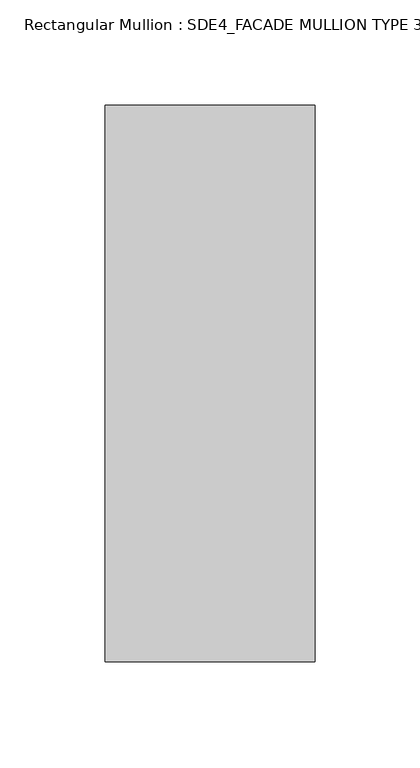
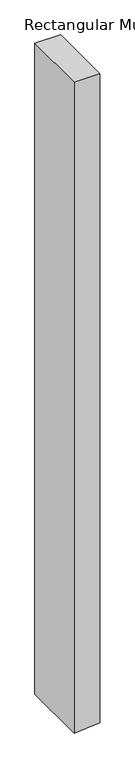
"""IFC4 building model written with IfcOpenShell, lengths in millimetres: member geometry, Rectangular Mullion : SDE4_FACADE MULLION TYPE 3."""

from ifc_helpers import new_model, si_unit, frame, origin, place, context, project, spatial, polyline, outline, extrude, source, transform, mapped, element, save


def rectangular_mullion_sde4_facade_mullion_type_3_780f94bb(model_context):
    return source(origin(), model_context, "Body", "SweptSolid", [
        extrude(outline(polyline([(0.0, 50.0), (0.0, -50.0), (-2678.1277723, -50.0), (-2674.530175, -3.056508), (-2670.4640959, 50.0), (0.0, 50.0)])), frame((0.0, -132.5, 0.0), z_axis=(0.0, 1.0, 0.0), x_axis=(0.0, 0.0, 1.0)), (0.0, 0.0, 1.0), 265.0),
    ])


if __name__ == "__main__":
    model = new_model("IFC4")
    model_context = context("Model", 3, world=origin())
    ifc_project = project(units=[si_unit("LENGTHUNIT", "METRE", prefix="MILLI")], contexts=[model_context])
    site = spatial("IfcSite", under=ifc_project)
    building = spatial("IfcBuilding", under=site)
    placement = place(None, origin())
    rectangular_mullion_sde4_facade_mullion_type_3_shape = rectangular_mullion_sde4_facade_mullion_type_3_780f94bb(model_context)
    element("IfcMember", 1, ObjectType="Rectangular Mullion : SDE4_FACADE MULLION TYPE 3", at=placement, inside=building, context=model_context, shape_type="MappedRepresentation", body=[
        mapped(rectangular_mullion_sde4_facade_mullion_type_3_shape, transform((0.0, 0.0, 0.0), x_axis=(1.0, 0.0, 0.0), y_axis=(0.0, 1.0, 0.0), z_axis=(0.0, 0.0, 1.0))),
    ])
    save(model, "model.ifc")

# Revit data of these elements
# Type "Rectangular Mullion : SDE4_FACADE MULLION TYPE 3"
#   built-in parameter 1007322 = 0.869423 (stored number, unit not read)
#   built-in parameter 1007321 = 0.164042 (stored number, unit not read)
#   built-in parameter 1007320 = 0.164042 (stored number, unit not read)
